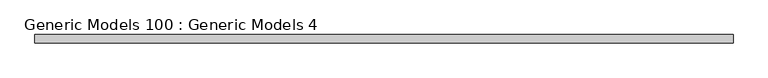
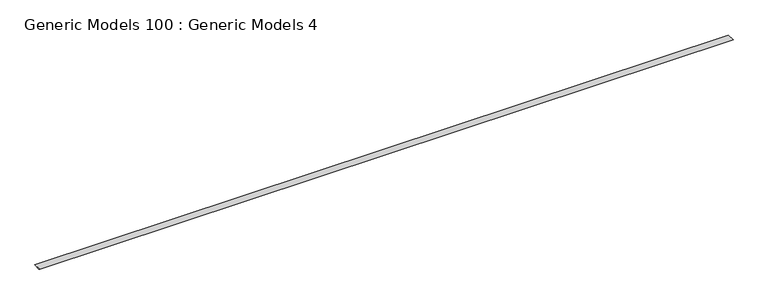
"""IFC4 building model written with IfcOpenShell, lengths in millimetres: proxy geometry, Generic Models 100 : Generic Models 4."""

import ifcopenshell
import ifcopenshell.guid

model = None  # the IFC model being written
_history = None  # IfcOwnerHistory: only IFC2X3 demands one
_inside = {}  # id of a spatial element -> (the spatial element, [elements in it])
_under = {}  # id of a project, library or spatial element -> (it, [spatial elements below it])
_declared = {}  # id of a project -> (the project, [libraries it declares])
_typed = {}  # id of a type object -> (the type object, [elements of that type])
_made_of = {}  # id of a material, layer set ... -> (it, [elements and type objects made of it])


def new_model(schema):
    """Start an empty IFC model of exactly this schema.

    Asked for "IFC4X3", IfcOpenShell would pick the latest addendum, in which some entities
    have other attributes; the version numbers below select the first issue.
    IFC2X3 requires an IfcOwnerHistory on every rooted entity: one is made here for all.
    """
    global model, _history
    if schema == "IFC4X3":
        model = ifcopenshell.file(schema_version=(4, 3, 0, 0))
    else:
        model = ifcopenshell.file(schema=schema)
    _inside.clear()
    _under.clear()
    _declared.clear()
    _typed.clear()
    _made_of.clear()
    _history = None
    if model.schema == "IFC2X3":
        org = make("IfcOrganization", Name="unknown")
        user = make(
            "IfcPersonAndOrganization",
            ThePerson=make("IfcPerson", FamilyName="unknown"),
            TheOrganization=org,
        )
        app = make(
            "IfcApplication",
            ApplicationDeveloper=org,
            Version="unknown",
            ApplicationFullName="unknown",
            ApplicationIdentifier="unknown",
        )
        _history = make(
            "IfcOwnerHistory",
            OwningUser=user,
            OwningApplication=app,
            ChangeAction="ADDED",
            CreationDate=0,
        )
    return model


def make(cls, **values):
    """One entity of the class cls with the attributes given. An attribute that is None is left unset."""
    return model.create_entity(
        cls, **{name: value for name, value in values.items() if value is not None}
    )


def rooted(cls, **values):
    """An entity with a GlobalId (a new one), such as an element, a storey or a relation."""
    return make(cls, GlobalId=ifcopenshell.guid.new(), OwnerHistory=_history, **values)


def si_unit(unit_type, name, prefix=None):
    """IfcSIUnit, for example si_unit("LENGTHUNIT", "METRE", prefix="MILLI")."""
    return make("IfcSIUnit", UnitType=unit_type, Prefix=prefix, Name=name)


def assignment(units):
    """IfcUnitAssignment: the units of a project."""
    return None if units is None else make("IfcUnitAssignment", Units=units)


def point(xyz):
    """IfcCartesianPoint."""
    return None if xyz is None else make("IfcCartesianPoint", Coordinates=xyz)


def direction(xyz):
    """IfcDirection."""
    return None if xyz is None else make("IfcDirection", DirectionRatios=xyz)


def frame(location, z_axis=None, x_axis=None):
    """IfcAxis2Placement3D, a coordinate frame: its origin and axes. An axis left out is left unset."""
    return make(
        "IfcAxis2Placement3D",
        Location=point(location),
        Axis=direction(z_axis),
        RefDirection=direction(x_axis),
    )


def origin():
    """The frame at (0, 0, 0) with its axes left unset."""
    return frame((0.0, 0.0, 0.0))


def place(relative_to, where):
    """IfcLocalPlacement: puts the frame where relative to a parent placement (None: the world)."""
    return make(
        "IfcLocalPlacement", PlacementRelTo=relative_to, RelativePlacement=where
    )


def context(
    kind, dimensions, precision=None, world=None, true_north=None, identifier=None
):
    """IfcGeometricRepresentationContext, for example the 3D "Model" context."""
    return make(
        "IfcGeometricRepresentationContext",
        ContextIdentifier=identifier,
        ContextType=kind,
        CoordinateSpaceDimension=dimensions,
        Precision=precision,
        WorldCoordinateSystem=world,
        TrueNorth=true_north,
    )


def project(units=None, contexts=None):
    """IfcProject with its units and contexts."""
    return rooted(
        "IfcProject",
        Name="project",
        RepresentationContexts=contexts,
        UnitsInContext=assignment(units),
    )


def spatial(cls, under=None, at=None, **own):
    """A site, building, storey or space (cls), placed at a placement, below another one or the project."""
    s = rooted(cls, ObjectPlacement=at, **own)
    if under is not None:
        _under.setdefault(under.id(), (under, []))[1].append(s)
    return s


def polyline(points):
    """IfcPolyline through the points."""
    return make("IfcPolyline", Points=[point(p) for p in points])


def outline(outer, holes=None, kind="AREA"):
    """IfcArbitraryClosedProfileDef: a profile drawn as a closed curve; with holes, ...WithVoids."""
    if holes is None:
        return make("IfcArbitraryClosedProfileDef", ProfileType=kind, OuterCurve=outer)
    return make(
        "IfcArbitraryProfileDefWithVoids",
        ProfileType=kind,
        OuterCurve=outer,
        InnerCurves=holes,
    )


def extrude(swept, where, along, depth):
    """IfcExtrudedAreaSolid: the profile swept, set in the frame where, extruded along a direction by depth."""
    return make(
        "IfcExtrudedAreaSolid",
        SweptArea=swept,
        Position=where,
        ExtrudedDirection=direction(along),
        Depth=depth,
    )


def shape(context_of_items, identifier, shape_type, items):
    """IfcShapeRepresentation: the items that make up one representation, for example the "Body"."""
    return make(
        "IfcShapeRepresentation",
        ContextOfItems=context_of_items,
        RepresentationIdentifier=identifier,
        RepresentationType=shape_type,
        Items=items,
    )


def source(mapping_origin, context_of_items, identifier, shape_type, items):
    """IfcRepresentationMap: a shape defined once, which mapped items show again and again."""
    return make(
        "IfcRepresentationMap",
        MappingOrigin=mapping_origin,
        MappedRepresentation=shape(context_of_items, identifier, shape_type, items),
    )


def transform(
    local_origin,
    x_axis=None,
    y_axis=None,
    z_axis=None,
    scale=None,
    scale2=None,
    scale3=None,
    uniform=True,
):
    """IfcCartesianTransformationOperator3D, or its non-uniform kind. x_axis, y_axis, z_axis: its Axis1, 2, 3."""
    if uniform:
        return make(
            "IfcCartesianTransformationOperator3D",
            Axis1=direction(x_axis),
            Axis2=direction(y_axis),
            LocalOrigin=point(local_origin),
            Scale=scale,
            Axis3=direction(z_axis),
        )
    return make(
        "IfcCartesianTransformationOperator3DnonUniform",
        Axis1=direction(x_axis),
        Axis2=direction(y_axis),
        LocalOrigin=point(local_origin),
        Scale=scale,
        Axis3=direction(z_axis),
        Scale2=scale2,
        Scale3=scale3,
    )


def mapped(mapping_source, mapping_target):
    """IfcMappedItem: shows the shape of a source again, moved by a transform."""
    return make(
        "IfcMappedItem", MappingSource=mapping_source, MappingTarget=mapping_target
    )


def made_of(thing, what):
    """Note that an element or type object is made of a material, layer set ...; save() writes the relation."""
    if what is not None:
        _made_of.setdefault(what.id(), (what, []))[1].append(thing)
    return thing


def element(
    cls,
    number,
    at=None,
    inside=None,
    cuts=None,
    type_object=None,
    material=None,
    context=None,
    identifier="Body",
    shape_type=None,
    held_by="IfcProductDefinitionShape",
    body=None,
    shapes=None,
    **own,
):
    """One element of the class cls, such as IfcWall. Its Tag is "e" and its number.

    at: its placement. inside: the storey or other place that contains it. cuts: it is an
    opening in that element (IfcRelVoidsElement). A single representation is given by context,
    identifier, shape_type and body (its items); several are given by shapes. held_by: the class
    of the entity that holds the representations. save() writes the other relations.
    """
    e = rooted(cls, Tag="e%d" % number, ObjectPlacement=at, **own)
    if body is not None:
        shapes = [shape(context, identifier, shape_type, body)]
    if shapes is not None:
        e.Representation = make(held_by, Representations=shapes)
    if inside is not None:
        _inside.setdefault(inside.id(), (inside, []))[1].append(e)
    if cuts is not None:
        rooted(
            "IfcRelVoidsElement", RelatingBuildingElement=cuts, RelatedOpeningElement=e
        )
    if type_object is not None:
        _typed.setdefault(type_object.id(), (type_object, []))[1].append(e)
    return made_of(e, material)


def aggregate(whole, parts):
    """IfcRelAggregates: a whole, such as a stair, and the parts it consists of."""
    return rooted("IfcRelAggregates", RelatingObject=whole, RelatedObjects=parts)


def save(model, path):
    """Write the relations noted so far, then the file.

    IfcRelAggregates (storeys below a building ...), IfcRelContainedInSpatialStructure (elements
    in a storey), IfcRelDefinesByType, IfcRelAssociatesMaterial and IfcRelDeclares: one each for
    every whole, place, type object, material and project.
    """
    for whole, parts in _under.values():
        aggregate(whole, parts)
    for where, things in _inside.values():
        rooted(
            "IfcRelContainedInSpatialStructure",
            RelatedElements=things,
            RelatingStructure=where,
        )
    for kind, things in _typed.values():
        rooted("IfcRelDefinesByType", RelatedObjects=things, RelatingType=kind)
    for what, things in _made_of.values():
        rooted("IfcRelAssociatesMaterial", RelatedObjects=things, RelatingMaterial=what)
    for by, libraries in _declared.values():
        rooted("IfcRelDeclares", RelatingContext=by, RelatedDefinitions=libraries)
    model.write(path)


def generic_models_100_generic_models_4_4776cf9e(model_context):
    return source(origin(), model_context, "Body", "SweptSolid", [
        extrude(outline(polyline([(7044.4437111, 127124.338344), (6889.0631112, 127127.5230447), (6852.9919, 127146.0460991), (7077.7459829, 127141.4395105), (7044.4437111, 127124.338344)])), frame((-10234.5171316, 0.0, 0.0), z_axis=(1.0, 0.0, 0.0), x_axis=(0.0, 1.0, 0.0)), (0.0, 0.0, 1.0), 18643.6),
    ])


if __name__ == "__main__":
    model = new_model("IFC4")
    model_context = context("Model", 3, world=origin())
    ifc_project = project(units=[si_unit("LENGTHUNIT", "METRE", prefix="MILLI")], contexts=[model_context])
    site = spatial("IfcSite", under=ifc_project)
    building = spatial("IfcBuilding", under=site)
    placement = place(None, origin())
    generic_models_100_generic_models_4_shape = generic_models_100_generic_models_4_4776cf9e(model_context)
    element("IfcBuildingElementProxy", 1, Name="Generic Models 100 : Generic Models 4", ObjectType="Generic Models 100 : Generic Models 4", at=placement, inside=building, context=model_context, shape_type="MappedRepresentation", body=[
        mapped(generic_models_100_generic_models_4_shape, transform((0.0, 0.0, 0.0), x_axis=(1.0, 0.0, 0.0), y_axis=(0.0, 1.0, 0.0), z_axis=(0.0, 0.0, 1.0))),
    ])
    save(model, "model.ifc")

# Revit data of these elements
# Element 1 (IfcBuildingElementProxy, "Generic Models 100 : Generic Models 4")
#   Materials on its faces: "_7/8\" SMOOTH TROWEL EXTERIOR STUCCO (COLOR PER OWNER) @ 2% SLOPE"
# Materials
#   "_7/8\" SMOOTH TROWEL EXTERIOR STUCCO (COLOR PER OWNER) @ 2% SLOPE": class "Generic", colour RGB 233 233 233, transparency 0, Cost = 0
